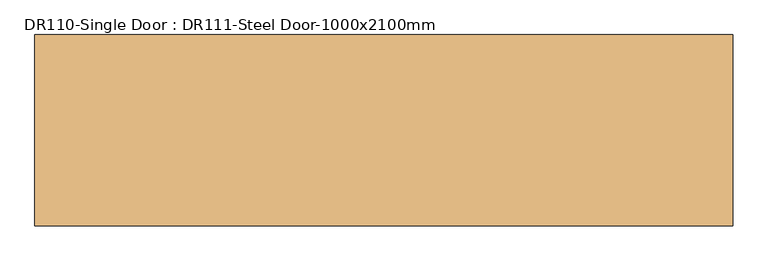
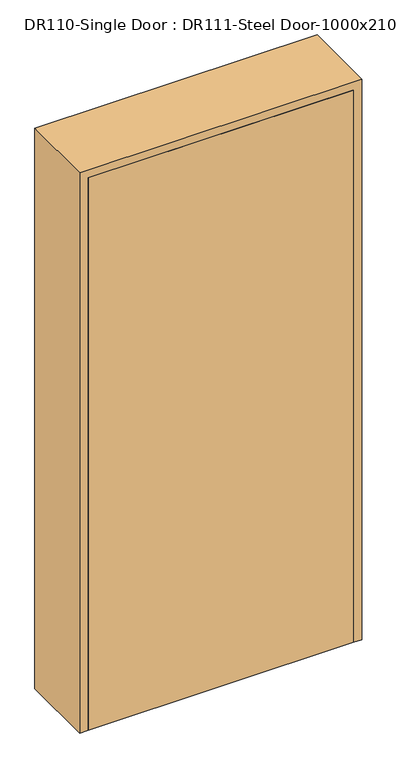
"""IFC4 building model written with IfcOpenShell, lengths in millimetres: door geometry, DR110-Single Door : DR111-Steel Door-1000x2100mm."""

import ifcopenshell
import ifcopenshell.guid

model = None  # the IFC model being written
_history = None  # IfcOwnerHistory: only IFC2X3 demands one
_inside = {}  # id of a spatial element -> (the spatial element, [elements in it])
_under = {}  # id of a project, library or spatial element -> (it, [spatial elements below it])
_declared = {}  # id of a project -> (the project, [libraries it declares])
_typed = {}  # id of a type object -> (the type object, [elements of that type])
_made_of = {}  # id of a material, layer set ... -> (it, [elements and type objects made of it])


def new_model(schema):
    """Start an empty IFC model of exactly this schema.

    Asked for "IFC4X3", IfcOpenShell would pick the latest addendum, in which some entities
    have other attributes; the version numbers below select the first issue.
    IFC2X3 requires an IfcOwnerHistory on every rooted entity: one is made here for all.
    """
    global model, _history
    if schema == "IFC4X3":
        model = ifcopenshell.file(schema_version=(4, 3, 0, 0))
    else:
        model = ifcopenshell.file(schema=schema)
    _inside.clear()
    _under.clear()
    _declared.clear()
    _typed.clear()
    _made_of.clear()
    _history = None
    if model.schema == "IFC2X3":
        org = make("IfcOrganization", Name="unknown")
        user = make(
            "IfcPersonAndOrganization",
            ThePerson=make("IfcPerson", FamilyName="unknown"),
            TheOrganization=org,
        )
        app = make(
            "IfcApplication",
            ApplicationDeveloper=org,
            Version="unknown",
            ApplicationFullName="unknown",
            ApplicationIdentifier="unknown",
        )
        _history = make(
            "IfcOwnerHistory",
            OwningUser=user,
            OwningApplication=app,
            ChangeAction="ADDED",
            CreationDate=0,
        )
    return model


def make(cls, **values):
    """One entity of the class cls with the attributes given. An attribute that is None is left unset."""
    return model.create_entity(
        cls, **{name: value for name, value in values.items() if value is not None}
    )


def rooted(cls, **values):
    """An entity with a GlobalId (a new one), such as an element, a storey or a relation."""
    return make(cls, GlobalId=ifcopenshell.guid.new(), OwnerHistory=_history, **values)


def si_unit(unit_type, name, prefix=None):
    """IfcSIUnit, for example si_unit("LENGTHUNIT", "METRE", prefix="MILLI")."""
    return make("IfcSIUnit", UnitType=unit_type, Prefix=prefix, Name=name)


def assignment(units):
    """IfcUnitAssignment: the units of a project."""
    return None if units is None else make("IfcUnitAssignment", Units=units)


def point(xyz):
    """IfcCartesianPoint."""
    return None if xyz is None else make("IfcCartesianPoint", Coordinates=xyz)


def direction(xyz):
    """IfcDirection."""
    return None if xyz is None else make("IfcDirection", DirectionRatios=xyz)


def frame(location, z_axis=None, x_axis=None):
    """IfcAxis2Placement3D, a coordinate frame: its origin and axes. An axis left out is left unset."""
    return make(
        "IfcAxis2Placement3D",
        Location=point(location),
        Axis=direction(z_axis),
        RefDirection=direction(x_axis),
    )


def origin():
    """The frame at (0, 0, 0) with its axes left unset."""
    return frame((0.0, 0.0, 0.0))


def origin_with_axes():
    """The frame at (0, 0, 0) with the z axis (0, 0, 1) and the x axis (1, 0, 0) written out."""
    return frame((0.0, 0.0, 0.0), z_axis=(0.0, 0.0, 1.0), x_axis=(1.0, 0.0, 0.0))


def place(relative_to, where):
    """IfcLocalPlacement: puts the frame where relative to a parent placement (None: the world)."""
    return make(
        "IfcLocalPlacement", PlacementRelTo=relative_to, RelativePlacement=where
    )


def context(
    kind, dimensions, precision=None, world=None, true_north=None, identifier=None
):
    """IfcGeometricRepresentationContext, for example the 3D "Model" context."""
    return make(
        "IfcGeometricRepresentationContext",
        ContextIdentifier=identifier,
        ContextType=kind,
        CoordinateSpaceDimension=dimensions,
        Precision=precision,
        WorldCoordinateSystem=world,
        TrueNorth=true_north,
    )


def project(units=None, contexts=None):
    """IfcProject with its units and contexts."""
    return rooted(
        "IfcProject",
        Name="project",
        RepresentationContexts=contexts,
        UnitsInContext=assignment(units),
    )


def spatial(cls, under=None, at=None, **own):
    """A site, building, storey or space (cls), placed at a placement, below another one or the project."""
    s = rooted(cls, ObjectPlacement=at, **own)
    if under is not None:
        _under.setdefault(under.id(), (under, []))[1].append(s)
    return s


def polyline(points):
    """IfcPolyline through the points."""
    return make("IfcPolyline", Points=[point(p) for p in points])


def outline(outer, holes=None, kind="AREA"):
    """IfcArbitraryClosedProfileDef: a profile drawn as a closed curve; with holes, ...WithVoids."""
    if holes is None:
        return make("IfcArbitraryClosedProfileDef", ProfileType=kind, OuterCurve=outer)
    return make(
        "IfcArbitraryProfileDefWithVoids",
        ProfileType=kind,
        OuterCurve=outer,
        InnerCurves=holes,
    )


def extrude(swept, where, along, depth):
    """IfcExtrudedAreaSolid: the profile swept, set in the frame where, extruded along a direction by depth."""
    return make(
        "IfcExtrudedAreaSolid",
        SweptArea=swept,
        Position=where,
        ExtrudedDirection=direction(along),
        Depth=depth,
    )


def faces_of(points, faces, orient=None, outer=None):
    """IfcFace entities. A face is a list of loops; a loop is a list of indices into points, from 0.

    orient and outer hold one flag for each loop. By default every Orientation is true, the
    first loop of a face is its IfcFaceOuterBound and the others are IfcFaceBound.
    """
    made = []
    for i, loops in enumerate(faces):
        bounds = []
        for j, loop in enumerate(loops):
            is_outer = j == 0 if outer is None else outer[i][j]
            bounds.append(
                make(
                    "IfcFaceOuterBound" if is_outer else "IfcFaceBound",
                    Bound=make("IfcPolyLoop", Polygon=[points[k] for k in loop]),
                    Orientation=True if orient is None else orient[i][j],
                )
            )
        made.append(make("IfcFace", Bounds=bounds))
    return made


def faceted_brep(points, faces, orient=None, outer=None, voids=None):
    """IfcFacetedBrep: a solid bounded by flat faces; with voids (closed shells), ...WithVoids."""
    shared = [point(p) for p in points]
    hull = make("IfcClosedShell", CfsFaces=faces_of(shared, faces, orient, outer))
    if voids is None:
        return make("IfcFacetedBrep", Outer=hull)
    return make(
        "IfcFacetedBrepWithVoids",
        Outer=hull,
        Voids=[
            make(cls, CfsFaces=faces_of(shared, fs, o, b)) for cls, fs, o, b in voids
        ],
    )


def shape(context_of_items, identifier, shape_type, items):
    """IfcShapeRepresentation: the items that make up one representation, for example the "Body"."""
    return make(
        "IfcShapeRepresentation",
        ContextOfItems=context_of_items,
        RepresentationIdentifier=identifier,
        RepresentationType=shape_type,
        Items=items,
    )


def source(mapping_origin, context_of_items, identifier, shape_type, items):
    """IfcRepresentationMap: a shape defined once, which mapped items show again and again."""
    return make(
        "IfcRepresentationMap",
        MappingOrigin=mapping_origin,
        MappedRepresentation=shape(context_of_items, identifier, shape_type, items),
    )


def transform(
    local_origin,
    x_axis=None,
    y_axis=None,
    z_axis=None,
    scale=None,
    scale2=None,
    scale3=None,
    uniform=True,
):
    """IfcCartesianTransformationOperator3D, or its non-uniform kind. x_axis, y_axis, z_axis: its Axis1, 2, 3."""
    if uniform:
        return make(
            "IfcCartesianTransformationOperator3D",
            Axis1=direction(x_axis),
            Axis2=direction(y_axis),
            LocalOrigin=point(local_origin),
            Scale=scale,
            Axis3=direction(z_axis),
        )
    return make(
        "IfcCartesianTransformationOperator3DnonUniform",
        Axis1=direction(x_axis),
        Axis2=direction(y_axis),
        LocalOrigin=point(local_origin),
        Scale=scale,
        Axis3=direction(z_axis),
        Scale2=scale2,
        Scale3=scale3,
    )


def mapped(mapping_source, mapping_target):
    """IfcMappedItem: shows the shape of a source again, moved by a transform."""
    return make(
        "IfcMappedItem", MappingSource=mapping_source, MappingTarget=mapping_target
    )


def made_of(thing, what):
    """Note that an element or type object is made of a material, layer set ...; save() writes the relation."""
    if what is not None:
        _made_of.setdefault(what.id(), (what, []))[1].append(thing)
    return thing


def element(
    cls,
    number,
    at=None,
    inside=None,
    cuts=None,
    type_object=None,
    material=None,
    context=None,
    identifier="Body",
    shape_type=None,
    held_by="IfcProductDefinitionShape",
    body=None,
    shapes=None,
    **own,
):
    """One element of the class cls, such as IfcWall. Its Tag is "e" and its number.

    at: its placement. inside: the storey or other place that contains it. cuts: it is an
    opening in that element (IfcRelVoidsElement). A single representation is given by context,
    identifier, shape_type and body (its items); several are given by shapes. held_by: the class
    of the entity that holds the representations. save() writes the other relations.
    """
    e = rooted(cls, Tag="e%d" % number, ObjectPlacement=at, **own)
    if body is not None:
        shapes = [shape(context, identifier, shape_type, body)]
    if shapes is not None:
        e.Representation = make(held_by, Representations=shapes)
    if inside is not None:
        _inside.setdefault(inside.id(), (inside, []))[1].append(e)
    if cuts is not None:
        rooted(
            "IfcRelVoidsElement", RelatingBuildingElement=cuts, RelatedOpeningElement=e
        )
    if type_object is not None:
        _typed.setdefault(type_object.id(), (type_object, []))[1].append(e)
    return made_of(e, material)


def aggregate(whole, parts):
    """IfcRelAggregates: a whole, such as a stair, and the parts it consists of."""
    return rooted("IfcRelAggregates", RelatingObject=whole, RelatedObjects=parts)


def save(model, path):
    """Write the relations noted so far, then the file.

    IfcRelAggregates (storeys below a building ...), IfcRelContainedInSpatialStructure (elements
    in a storey), IfcRelDefinesByType, IfcRelAssociatesMaterial and IfcRelDeclares: one each for
    every whole, place, type object, material and project.
    """
    for whole, parts in _under.values():
        aggregate(whole, parts)
    for where, things in _inside.values():
        rooted(
            "IfcRelContainedInSpatialStructure",
            RelatedElements=things,
            RelatingStructure=where,
        )
    for kind, things in _typed.values():
        rooted("IfcRelDefinesByType", RelatedObjects=things, RelatingType=kind)
    for what, things in _made_of.values():
        rooted("IfcRelAssociatesMaterial", RelatedObjects=things, RelatingMaterial=what)
    for by, libraries in _declared.values():
        rooted("IfcRelDeclares", RelatingContext=by, RelatedDefinitions=libraries)
    model.write(path)


def dr110_single_door_dr111_steel_door_1000x2100mm_c730d40a(model_context):
    return source(origin(), model_context, "Body", "SolidModel", [
        extrude(outline(polyline([(470.0, -137.0), (-470.0, -137.0), (-470.0, -102.0), (470.0, -102.0), (470.0, -137.0)])), origin_with_axes(), (0.0, 0.0, 1.0), 2070.0),
        faceted_brep([(470.0, -137.0, 0.0), (470.0, -102.0, 0.0), (450.0, -102.0, 0.0), (450.0, 102.0, 0.0), (470.0, 102.0, 0.0), (470.0, 137.0, 0.0), (500.0, 137.0, 0.0), (500.0, -137.0, 0.0), (500.0, -137.0, 2100.0), (-500.0, -137.0, 2100.0), (-500.0, -137.0, 0.0), (-470.0, -137.0, 0.0), (-470.0, -137.0, 2070.0), (470.0, -137.0, 2070.0), (500.0, 137.0, 2100.0), (470.0, 137.0, 2070.0), (-470.0, 137.0, 2070.0), (-470.0, 137.0, 0.0), (-500.0, 137.0, 0.0), (-500.0, 137.0, 2100.0), (470.0, 102.0, 2070.0), (450.0, 102.0, 2050.0), (-450.0, 102.0, 2050.0), (-450.0, 102.0, 0.0), (-470.0, 102.0, 0.0), (-470.0, 102.0, 2070.0), (450.0, -102.0, 2050.0), (470.0, -102.0, 2070.0), (-470.0, -102.0, 2070.0), (-470.0, -102.0, 0.0), (-450.0, -102.0, 0.0), (-450.0, -102.0, 2050.0)], [[[0, 1, 2, 3, 4, 5, 6, 7]], [[7, 8, 9, 10, 11, 12, 13, 0]], [[6, 14, 8, 7]], [[5, 15, 16, 17, 18, 19, 14, 6]], [[4, 20, 15, 5]], [[3, 21, 22, 23, 24, 25, 20, 4]], [[2, 26, 21, 3]], [[1, 27, 28, 29, 30, 31, 26, 2]], [[0, 13, 27, 1]], [[12, 11, 29, 28]], [[11, 10, 18, 17, 24, 23, 30, 29]], [[19, 18, 10, 9]], [[25, 24, 17, 16]], [[31, 30, 23, 22]], [[14, 19, 9, 8]], [[20, 25, 16, 15]], [[26, 31, 22, 21]], [[13, 12, 28, 27]]]),
    ])


if __name__ == "__main__":
    model = new_model("IFC4")
    model_context = context("Model", 3, world=origin())
    ifc_project = project(units=[si_unit("LENGTHUNIT", "METRE", prefix="MILLI")], contexts=[model_context])
    site = spatial("IfcSite", under=ifc_project)
    building = spatial("IfcBuilding", under=site)
    placement = place(None, origin())
    dr110_single_door_dr111_steel_door_1000x2100mm_shape = dr110_single_door_dr111_steel_door_1000x2100mm_c730d40a(model_context)
    element("IfcDoor", 1, ObjectType="DR110-Single Door : DR111-Steel Door-1000x2100mm", at=placement, inside=building, context=model_context, shape_type="MappedRepresentation", body=[
        mapped(dr110_single_door_dr111_steel_door_1000x2100mm_shape, transform((0.0, 0.0, 0.0), x_axis=(1.0, 0.0, 0.0), y_axis=(0.0, 1.0, 0.0), z_axis=(0.0, 0.0, 1.0))),
    ])
    save(model, "model.ifc")

# Revit data of these elements
# Type "DR110-Single Door : DR111-Steel Door-1000x2100mm"
#   Type Mark = "SD"
#   Analytic Construction = "<None>"
#   프레임 투영 외부. = 25 mm
#   프레임 투영 내부. = 25 mm
#   프레임 폭 = 75 mm
#   Height = 2100 mm
#   Width = 1000 mm
#   Define Thermal Properties by = 1
#   문 패널 = SD1 문 패널
#   문 프레임 = A04AQ098-00002_Steel Door_non FP_single
#   Function = (empty or 0)
#   Wall Closure = (empty or 0)
# Element 1 (IfcDoor, "DR110-Single Door : DR111-Steel Door-1000x2100mm")
#   Materials on its faces: "A04AQ098-00002_Steel Door_non FP_single", "SD1 문 패널"
# Materials
#   "SD1 문 패널": class "금속", colour RGB 247 247 247, transparency 0
#   "A04AQ098-00002_Steel Door_non FP_single": class "금속", colour RGB 247 247 247, transparency 0, Description = "Steel Door", W00) Work Master Code = "A04AQ098-00002", W01) Work Master_Lv1 = "Finishing Work", W02) Work Master_Lv2 = "Door & Window Work", W03) Work Master_Spec.1 = "Steel Door w/ Steel Frame", W04) Work Master_Spec.2 = "Fire Protective Rating: N/A, Single Door", W05) Work Master_Spec.3 = "w/ Hardware & Accessories", Cost = 0
